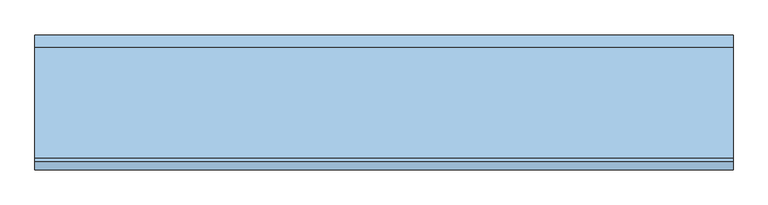
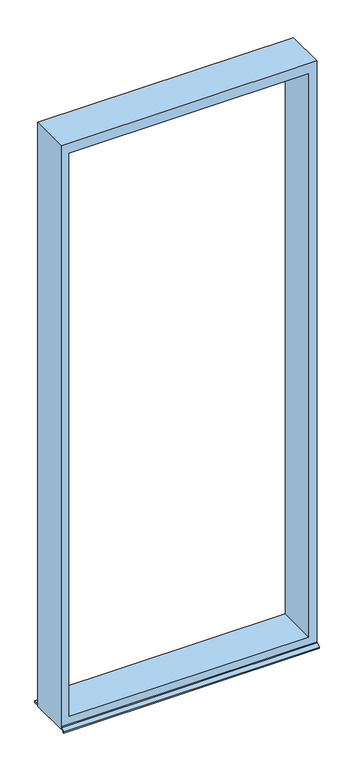
"""IFC4 building model written with IfcOpenShell, lengths in millimetres: window geometry, Fenster - Festverglasung : Feste Verglasung 4.58 x 1.9 2."""

from ifc_helpers import new_model, si_unit, frame, origin, place, context, project, spatial, polyline, outline, extrude, source, transform, mapped, element, save


def window_2efbcd40(model_context):
    return source(origin(), model_context, "Body", "SweptSolid", [
        extrude(outline(polyline([(5580.0, 950.0), (5580.0, -950.0), (1000.0, -950.0), (1000.0, 950.0), (5580.0, 950.0)]), holes=[polyline([(5500.0, 890.0), (1080.0, 890.0), (1080.0, -890.0), (5500.0, -890.0), (5500.0, 890.0)])]), frame((0.0, -151.5214598, 0.0), z_axis=(0.0, 1.0, 0.0), x_axis=(0.0, 0.0, 1.0)), (0.0, 0.0, 1.0), 300.0),
        extrude(outline(polyline([(-950.0, 184.0), (950.0, 184.0), (950.0, 148.4785402), (-950.0, 148.4785402), (-950.0, 184.0)])), frame((0.0, 0.0, 1005.0), z_axis=(0.0, 0.0, 1.0), x_axis=(1.0, 0.0, 0.0)), (0.0, 0.0, 1.0), 15.0),
        extrude(outline(polyline([(-161.5436142, 1020.0), (-151.5214598, 1020.0), (-151.5214598, 1018.0), (-161.3455321, 1018.0), (-182.0, 998.3604634), (-182.0, 990.0), (-184.0, 990.0), (-184.0, 1000.0), (-161.5436142, 1020.0)])), frame((-950.0, 0.0, 0.0), z_axis=(1.0, 0.0, 0.0), x_axis=(0.0, 1.0, 0.0)), (0.0, 0.0, 1.0), 1900.0),
    ])


if __name__ == "__main__":
    model = new_model("IFC4")
    model_context = context("Model", 3, world=origin())
    ifc_project = project(units=[si_unit("LENGTHUNIT", "METRE", prefix="MILLI")], contexts=[model_context])
    site = spatial("IfcSite", under=ifc_project)
    building = spatial("IfcBuilding", under=site)
    placement = place(None, origin())
    window_shape = window_2efbcd40(model_context)
    element("IfcWindow", 1, ObjectType="Fenster - Festverglasung : Feste Verglasung 4.58 x 1.9 2", at=placement, inside=building, context=model_context, shape_type="MappedRepresentation", body=[
        mapped(window_shape, transform((0.0, 0.0, 0.0), x_axis=(1.0, 0.0, 0.0), y_axis=(0.0, 1.0, 0.0), z_axis=(0.0, 0.0, 1.0))),
    ])
    save(model, "model.ifc")

# Revit data of these elements
# Type "Fenster - Festverglasung : Feste Verglasung 4.58 x 1.9 2"
#   Type Mark = "66"
#   Operation = "SinglePanel"
#   Keynote = "16.05.01"
#   Visual Light Transmittance = 0.9
#   Solar Heat Gain Coefficient = 0.78
#   Rough Width = 1.900 m
#   Rough Height = 4.580 m
#   Heat Transfer Coefficient (U) = 3.6886 W/(m²·K)
#   Rahmentiefe = 0.300 m
#   Rahmenhöhe unten = 0.080 m
#   Höhe oberer  Rahmen = 0.080 m
#   Rahmenbreite = 0.060 m
#   Height = 4.580 m
#   Einbautiefe (von außen) [instance default] = 0.080 m
#   Width = 1.900 m
#   Wall Closure = 3
#   Bild [instance default] = none
#   Glas [instance default] = none
#   Innere Fensterbank [instance default] = none
#   Äußere Fensterbank [instance default] = none
#   Construction Type Id = ""
#   Analytic Construction = (empty or 0)
# Element 1 (IfcWindow, "Fenster - Festverglasung : Feste Verglasung 4.58 x 1.9 2")
#   Einbautiefe (von außen) = 0.002479 m
#   Materials on its faces: "Kunststoff - Weiß", "Holz - Birke"
# Materials
#   "Kunststoff - Weiß": class "Kunststoff", colour RGB 249 249 249, transparency 0, Cost = 0
#   "Holz - Birke": class "Holz", colour RGB 213 164 103, transparency 0, Cost = 0
